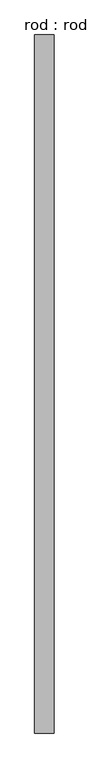
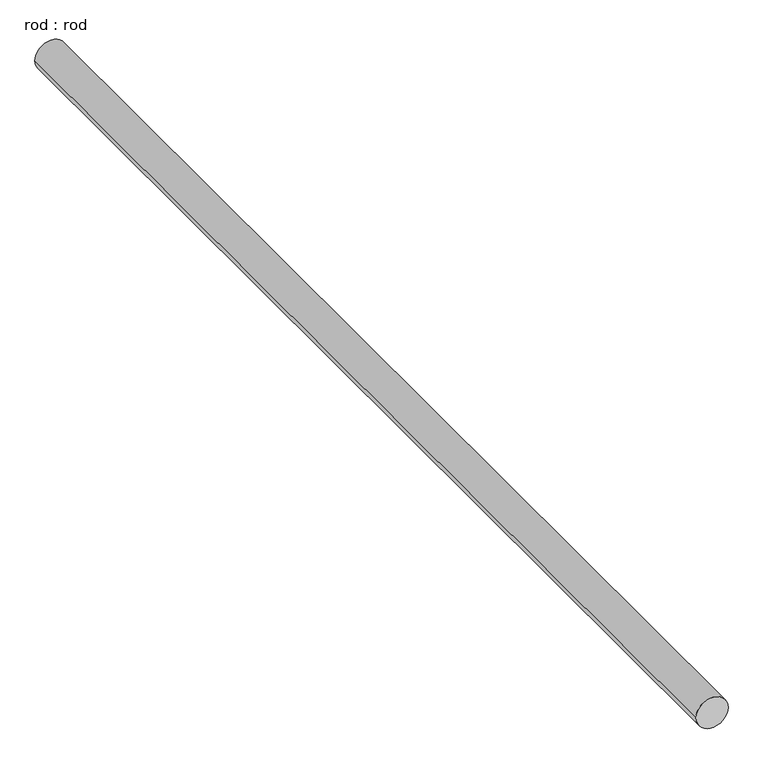
"""IFC4 building model written with IfcOpenShell, lengths in millimetres: proxy geometry, rod : rod."""

from ifc_helpers import new_model, si_unit, point, frame, frame_2d, origin, place, context, project, spatial, circle_curve, trimmed, segment, composite_curve, outline, extrude, source, transform, mapped, element, save


def rod_rod_fa39ebc7(model_context):
    return source(origin(), model_context, "Body", "SweptSolid", [
        extrude(outline(composite_curve([segment(trimmed(circle_curve(frame_2d((0.0108462, 0.0)), 200.0), [point((0.0108462, 200.0))], [point((0.0108462, -200.0))], False, "CARTESIAN"), True, "CONTINUOUS"), segment(trimmed(circle_curve(frame_2d((0.0108462, 0.0)), 200.0), [point((0.0108462, -200.0))], [point((0.0108462, 200.0))], False, "CARTESIAN"), True, "CONTINUOUS")], self_intersect=False)), frame((0.0, -3059.0570989, 0.0), z_axis=(0.0, 1.0, 0.0), x_axis=(0.0, 0.0, 1.0)), (0.0, 0.0, 1.0), 14303.5714286),
    ])


if __name__ == "__main__":
    model = new_model("IFC4")
    model_context = context("Model", 3, world=origin())
    ifc_project = project(units=[si_unit("LENGTHUNIT", "METRE", prefix="MILLI")], contexts=[model_context])
    site = spatial("IfcSite", under=ifc_project)
    building = spatial("IfcBuilding", under=site)
    placement = place(None, origin())
    rod_rod_shape = rod_rod_fa39ebc7(model_context)
    element("IfcBuildingElementProxy", 1, Name="rod : rod", ObjectType="rod : rod", at=placement, inside=building, context=model_context, shape_type="MappedRepresentation", body=[
        mapped(rod_rod_shape, transform((0.0, 0.0, 0.0), x_axis=(1.0, 0.0, 0.0), y_axis=(0.0, 1.0, 0.0), z_axis=(0.0, 0.0, 1.0))),
    ])
    save(model, "model.ifc")

# Revit data of these elements
# Type "rod : rod"
#   Default Elevation = 0
